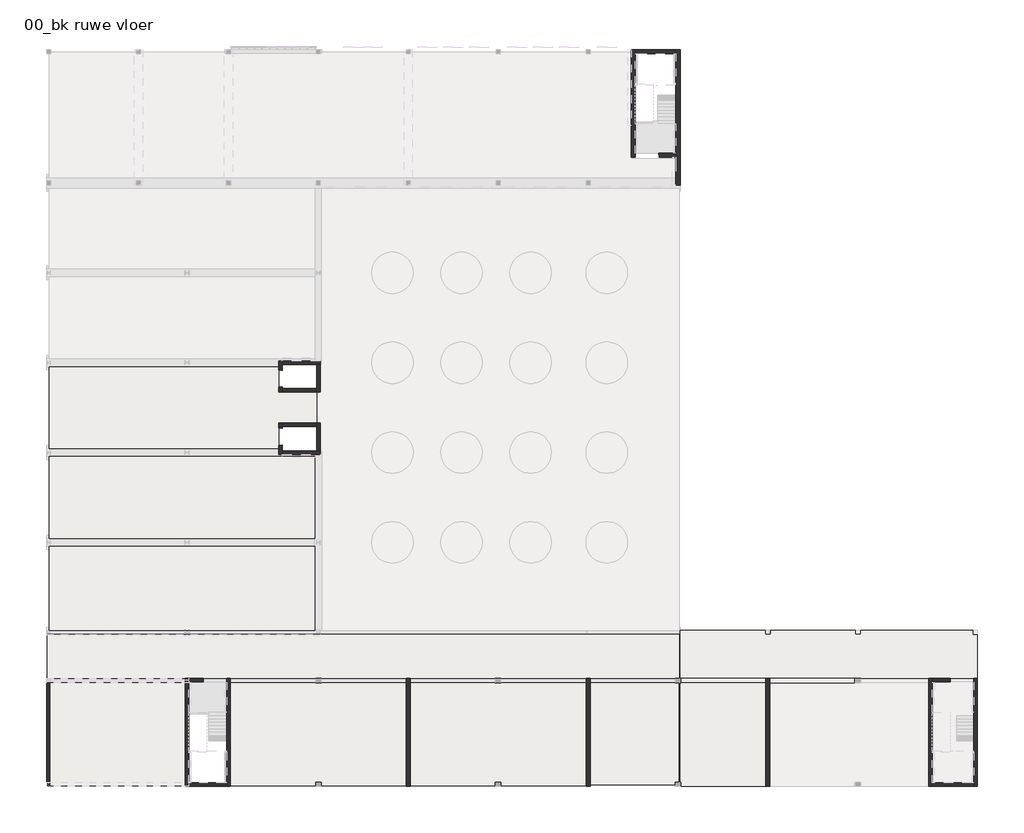
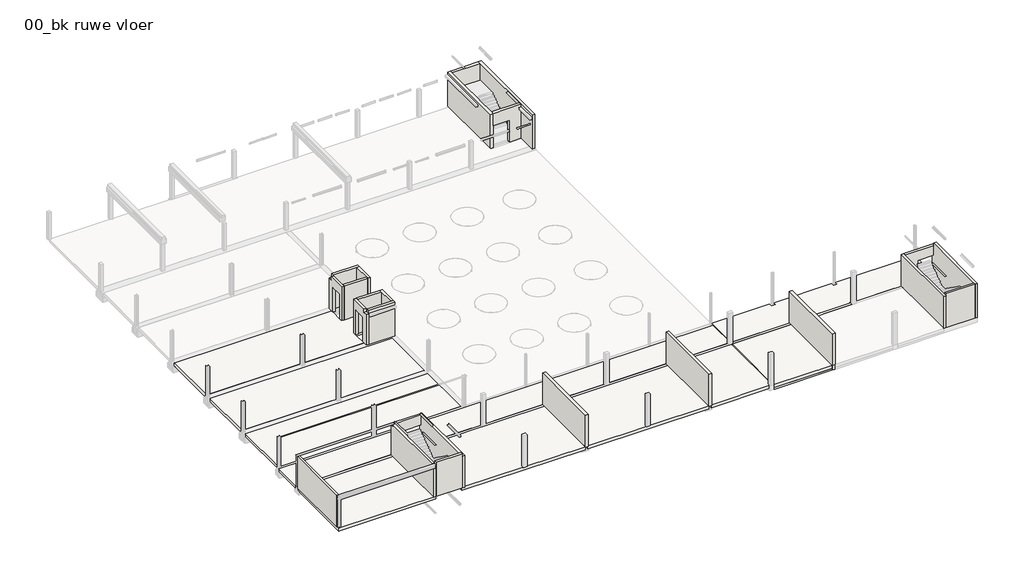
# One storey, part 1 of 6: 24 walls, 18 slabs.
# Revit data of these elements (continued)
# Element 20 (IfcWall, "NLRS_22_WA_beton ihw 250_gen_rsf") (continued)
#   IsExternal = no
#   LoadBearing = yes
#   Phase Created = NLRS_nieuw
#   Base Constraint = 00_bk ruwe vloer
#   Top Constraint = 01_ok ruwe vloer
#   Materials on its faces: "NLRS_f2_beton ihwg_gen_rsf"
# Element 21 (IfcWall, "NLRS_22_WA_kalkzandsteen CS20 300_gen_rsf")
#   IfcGUID = "03dfveMWnANRj9LlOnEnGT"
#   Comments = ""
#   Top Offset = 0 mm
#   Base Offset = 0 mm
#   wall height = 3540 mm
#   IsExternal = no
#   LoadBearing = yes
#   Phase Created = NLRS_nieuw
#   Base Constraint = 00_bk ruwe vloer
#   Top Constraint = 01_ok ruwe vloer
#   Materials on its faces: "NLRS_f1_kalkzandsteen_gen_rsf"
# Element 22 (IfcWall, "NLRS_22_WA_kalkzandsteen CS20 300_gen_rsf")
#   IfcGUID = "03dfveMWnANRj9LlOnEnH5"
#   Comments = ""
#   Top Offset = 0 mm
#   Base Offset = 0 mm
#   wall height = 3540 mm
#   IsExternal = no
#   LoadBearing = yes
#   Phase Created = NLRS_nieuw
#   Base Constraint = 00_bk ruwe vloer
#   Top Constraint = 01_ok ruwe vloer
#   Materials on its faces: "NLRS_f1_kalkzandsteen_gen_rsf"
# Element 23 (IfcWall, "NLRS_22_WA_kalkzandsteen CS20 300_gen_rsf")
#   IfcGUID = "03dfveMWnANRj9LlOnEnIp"
#   Comments = ""
#   Top Offset = 0 mm
#   Base Offset = 0 mm
#   wall height = 3540 mm
#   IsExternal = no
#   LoadBearing = yes
#   Phase Created = NLRS_nieuw
#   Base Constraint = 00_bk ruwe vloer
#   Top Constraint = 01_ok ruwe vloer
#   Materials on its faces: "NLRS_f1_kalkzandsteen_gen_rsf"
# Element 24 (IfcWall, "NLRS_21_WA_beton ihw 250_gen_rsf")
#   IfcGUID = "03dfveMWnANRj9LlOnEnKp"
#   Comments = ""
#   Top Offset = 0 mm
#   Base Offset = 0 mm
#   wall height = 3800 mm
#   IsExternal = yes
#   LoadBearing = yes
#   Phase Created = NLRS_nieuw
#   Base Constraint = 00_bk ruwe vloer
#   Top Constraint = 01_bk. ruwe vloer
#   Materials on its faces: "NLRS_f2_beton ihwg_gen_rsf"
# Element 25 (IfcWall, "NLRS_21_WA_kalkzandsteen CS12 214_gen_rsf")
#   IfcGUID = "2$hNzCXOT3YR8V$0Cfy_2r"
#   Comments = ""
#   Top Offset = 0 mm
#   Base Offset = 0 mm
#   wall height = 3540 mm
#   IsExternal = yes
#   LoadBearing = yes
#   Phase Created = NLRS_nieuw
#   Base Constraint = 00_bk ruwe vloer
#   Top Constraint = 01_ok ruwe vloer
#   Materials on its faces: "NLRS_f1_kalkzandsteen_gen_rsf"
# Element 26 (IfcWall, "NLRS_21_WA_beton ihw 250_gen_rsf")
#   IfcGUID = "2$hNzCXOT3YR8V$0Cfy_FB"
#   Top Offset = 0 mm
#   Base Offset = 0 mm
#   wall height = 3800 mm
#   IsExternal = yes
#   LoadBearing = yes
#   Phase Created = NLRS_nieuw
#   Base Constraint = 00_bk ruwe vloer
#   Top Constraint = 01_bk. ruwe vloer
#   Materials on its faces: "NLRS_f2_beton ihwg_gen_rsf"
# Element 27 (IfcWall, "NLRS_22_WA_beton ihw 250_gen_rsf")
#   IfcGUID = "2$hNzCXOT3YR8V$0Cfy_EM"
#   Top Offset = 0 mm
#   Base Offset = 0 mm
#   wall height = 3540 mm
#   IsExternal = no
#   LoadBearing = yes
#   Phase Created = NLRS_nieuw
#   Base Constraint = 00_bk ruwe vloer
#   Top Constraint = 01_ok ruwe vloer
#   Materials on its faces: "NLRS_f2_beton ihwg_gen_rsf"
# Element 28 (IfcWall, "NLRS_22_WA_beton ihw 250_gen_rsf")
#   IfcGUID = "2$hNzCXOT3YR8V$0Cfy_9A"
#   Comments = ""
#   Top Offset = 0 mm
#   Base Offset = 0 mm
#   wall height = 3540 mm
#   IsExternal = no
#   LoadBearing = yes
#   Phase Created = NLRS_nieuw
#   Base Constraint = 00_bk ruwe vloer
#   Top Constraint = 01_ok ruwe vloer
#   Materials on its faces: "NLRS_f2_beton ihwg_gen_rsf"
# Element 29 (IfcWall, "NLRS_21_WA_beton ihw 250_gen_rsf")
#   IfcGUID = "2$hNzCXOT3YR8V$0Cfy_84"
#   Top Offset = 0 mm
#   Base Offset = 0 mm
#   wall height = 3800 mm
#   IsExternal = yes
#   LoadBearing = yes
#   Phase Created = NLRS_nieuw
#   Base Constraint = 00_bk ruwe vloer
#   Top Constraint = 01_bk. ruwe vloer
#   Materials on its faces: "NLRS_f2_beton ihwg_gen_rsf"
# Element 30 (IfcWall, "NLRS_22_WA_beton ihw 250_gen_rsf")
#   IfcGUID = "2$hNzCXOT3YR8V$0Cfyzto"
#   Top Offset = 0 mm
#   Base Offset = 0 mm
#   wall height = 3540 mm
#   IsExternal = no
#   LoadBearing = yes
#   Phase Created = NLRS_nieuw
#   Base Constraint = 00_bk ruwe vloer
#   Top Constraint = 01_ok ruwe vloer
#   Materials on its faces: "NLRS_f2_beton ihwg_gen_rsf"
# Element 31 (IfcWall, "NLRS_22_WA_beton prefab 300_gen_rsf")
#   IfcGUID = "2ajLwCSRTE_9I1Spg4sCqL"
#   Comments = ""
#   built-in parameter 1001111 = 20 mm
#   Top Offset = 0 mm
#   Base Offset = 20 mm
#   wall height = 3780 mm
#   IsExternal = no
#   LoadBearing = yes
#   Phase Created = NLRS_nieuw
#   Base Constraint = 00_bk ruwe vloer
#   Top Constraint = 01_bk. ruwe vloer
#   Materials on its faces: "NLRS_f2_beton prefab_gen_rsf"
# Element 32 (IfcWall, "NLRS_21_WA_beton prefab 300_gen_rsf")
#   IfcGUID = "2ajLwCSRTE_9I1Spg4sCb7"
#   Comments = ""
#   built-in parameter 1001111 = 20 mm
#   Top Offset = 0 mm
#   Base Offset = 20 mm
#   wall height = 3780 mm
#   IsExternal = yes
#   LoadBearing = yes
#   Phase Created = NLRS_nieuw
#   Base Constraint = 00_bk ruwe vloer
#   Top Constraint = 01_bk. ruwe vloer
#   Materials on its faces: "NLRS_f2_beton prefab_gen_rsf"
# Element 33 (IfcWall, "NLRS_21_WA_beton prefab 300_gen_rsf")
#   IfcGUID = "2ajLwCSRTE_9I1Spg4sCao"
#   Comments = ""
#   built-in parameter 1001111 = 20 mm
#   Top Offset = 0 mm
#   Base Offset = 20 mm
#   wall height = 3780 mm
#   IsExternal = yes
#   LoadBearing = yes
#   Phase Created = NLRS_nieuw
#   Base Constraint = 00_bk ruwe vloer
#   Top Constraint = 01_bk. ruwe vloer
#   Materials on its faces: "NLRS_f2_beton prefab_gen_rsf"
# Element 34 (IfcWall, "NLRS_22_WA_beton prefab 300_gen_rsf")
#   IfcGUID = "2ajLwCSRTE_9I1Spg4sCWv"
#   Comments = ""
#   built-in parameter 1001111 = 20 mm
#   Top Offset = 0 mm
#   Base Offset = 20 mm
#   wall height = 3780 mm
#   IsExternal = no
#   LoadBearing = yes
#   Phase Created = NLRS_nieuw
#   Base Constraint = 00_bk ruwe vloer
#   Top Constraint = 01_bk. ruwe vloer
#   Materials on its faces: "NLRS_f2_beton prefab_gen_rsf"
# Element 35 (IfcWall, "NLRS_22_WA_beton prefab 250_gen_rsf")
#   IfcGUID = "2GRbcre991teoKeCLB8LzY"
#   built-in parameter 1001111 = 30 mm
#   Top Offset = 0 mm
#   Base Offset = 30 mm
#   wall height = 3770 mm
#   IsExternal = no
#   LoadBearing = yes
#   Phase Created = NLRS_nieuw
#   Base Constraint = 00_bk ruwe vloer
#   Top Constraint = 01_bk. ruwe vloer
#   Materials on its faces: "NLRS_f2_beton prefab_gen_rsf"
# Element 36 (IfcWall, "NLRS_22_WA_beton prefab 250_gen_rsf")
#   IfcGUID = "2GRbcre991teoKeCLB8Lp2"
#   built-in parameter 1001111 = 30 mm
#   Top Offset = 0 mm
#   Base Offset = 30 mm
#   wall height = 3770 mm
#   IsExternal = no
#   LoadBearing = yes
#   Phase Created = NLRS_nieuw
#   Base Constraint = 00_bk ruwe vloer
#   Top Constraint = 01_bk. ruwe vloer
#   Materials on its faces: "NLRS_f2_beton prefab_gen_rsf"
# Element 37 (IfcWall, "NLRS_22_WA_beton prefab 250_gen_rsf")
#   IfcGUID = "2GRbcre991teoKeCLB8LoQ"
#   built-in parameter 1001111 = 30 mm
#   Top Offset = 0 mm
#   Base Offset = 30 mm
#   wall height = 3770 mm
#   IsExternal = no
#   LoadBearing = yes
#   Phase Created = NLRS_nieuw
#   Base Constraint = 00_bk ruwe vloer
#   Top Constraint = 01_bk. ruwe vloer
#   Materials on its faces: "NLRS_f2_beton prefab_gen_rsf"
# Element 38 (IfcWall, "NLRS_21_WA_beton prefab 250_gen_rsf")
#   IfcGUID = "2GRbcre991teoKeCLB8LnQ"
#   built-in parameter 1001111 = 30 mm
#   Top Offset = 0 mm
#   Base Offset = 30 mm
#   wall height = 3770 mm
#   IsExternal = yes
#   LoadBearing = yes
#   Phase Created = NLRS_nieuw
#   Base Constraint = 00_bk ruwe vloer
#   Top Constraint = 01_bk. ruwe vloer
#   Materials on its faces: "NLRS_f2_beton prefab_gen_rsf"
# Element 39 (IfcWall, "NLRS_22_WA_beton prefab 250_gen_rsf")
#   IfcGUID = "2GRbcre991teoKeCLB8Lfd"
#   built-in parameter 1001111 = 30 mm
#   Top Offset = 0 mm
#   Base Offset = 30 mm
#   wall height = 3770 mm
#   IsExternal = no
#   LoadBearing = yes
#   Phase Created = NLRS_nieuw
#   Base Constraint = 00_bk ruwe vloer
#   Top Constraint = 01_bk. ruwe vloer
#   Materials on its faces: "NLRS_f2_beton prefab_gen_rsf"
# Element 40 (IfcWall, "NLRS_22_WA_beton prefab 250_gen_rsf")
#   IfcGUID = "2GRbcre991teoKeCLB8Lfb"
#   built-in parameter 1001111 = 30 mm
#   Top Offset = 0 mm
#   Base Offset = 30 mm
#   wall height = 3770 mm
#   IsExternal = no
#   LoadBearing = yes
#   Phase Created = NLRS_nieuw
#   Base Constraint = 00_bk ruwe vloer
#   Top Constraint = 01_bk. ruwe vloer
#   Materials on its faces: "NLRS_f2_beton prefab_gen_rsf"
# Element 41 (IfcWall, "NLRS_22_WA_beton prefab 250_gen_rsf")
#   IfcGUID = "2GRbcre991teoKeCLB8LfZ"
#   built-in parameter 1001111 = 30 mm
#   Top Offset = 0 mm
#   Base Offset = 30 mm
#   wall height = 3770 mm
#   IsExternal = no
#   LoadBearing = yes
#   Phase Created = NLRS_nieuw
#   Base Constraint = 00_bk ruwe vloer
#   Top Constraint = 01_bk. ruwe vloer
#   Materials on its faces: "NLRS_f2_beton prefab_gen_rsf"
# Element 42 (IfcWall, "NLRS_21_WA_beton prefab 250_gen_rsf")
#   IfcGUID = "2GRbcre991teoKeCLB8LfX"
#   built-in parameter 1001111 = 30 mm
#   Top Offset = 0 mm
#   Base Offset = 30 mm
#   wall height = 3770 mm
#   IsExternal = yes
#   LoadBearing = yes
#   Phase Created = NLRS_nieuw
#   Base Constraint = 00_bk ruwe vloer
#   Top Constraint = 01_bk. ruwe vloer
#   Materials on its faces: "NLRS_f2_beton prefab_gen_rsf"
# Materials
#   "NLRS_f2_beton prefab_gen_rsf": class "F - Niet gebakken kunststeen", colour RGB 129 133 118, transparency 0, Keynote = "f2", Manufacturer = "Revit Standards Foundation", URL = "www.revitstandards.org", Description = "beton prefab", Cost = 0
#   "NLRS_f2_beton ihwg_gen_rsf": class "F - Niet gebakken kunststeen", colour RGB 129 133 118, transparency 0, Keynote = "f2", Manufacturer = "Revit Standards Foundation", URL = "www.revitstandards.org", Description = "beton ihwg", Cost = 0
#   "NLRS_n7_isolatie EPS_gen_rsf": class "N - Kunststoffen, rubbers", colour RGB 200 200 140, transparency 0, Keynote = "n7", Manufacturer = "Revit Standards Foundation", URL = "www.revitstandards.org", Description = "isolatie EPS", Cost = 0
#   "NLRS_f1_kalkzandsteen_gen_rsf": class "F - Niet gebakken kunststeen", colour RGB 223 221 219, transparency 0, Keynote = "f1", Manufacturer = "Revit Standards Foundation", URL = "www.revitstandards.org", Description = "kalkzandsteen", Cost = 0
# Room, not placed, phase "NLRS_bestaand", upper offset 0 mm, lower offset 0 mm
#   Number = "1"
#   Name = "Room"
